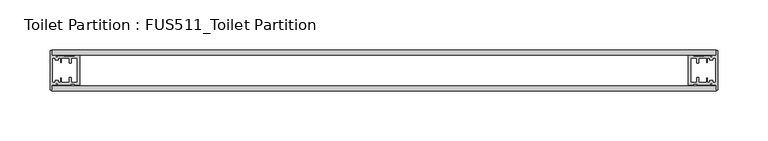
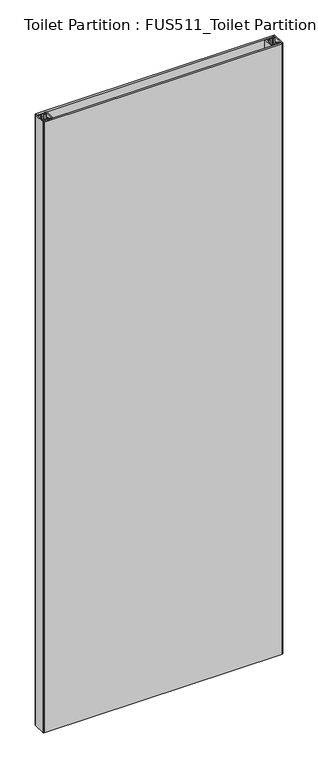
"""IFC4 building model written with IfcOpenShell, lengths in millimetres: furniture geometry, Toilet Partition : FUS511_Toilet Partition."""

from ifc_helpers import new_model, si_unit, point, frame, frame_2d, origin, place, context, project, spatial, polyline, circle_curve, trimmed, segment, composite_curve, outline, extrude, source, transform, mapped, element, save


def toilet_partition_fus511_toilet_partition_6d0bb69f(model_context):
    return source(origin(), model_context, "Body", "SweptSolid", [
        extrude(outline(composite_curve([segment(polyline([(-316.5997483, 489.5206414), (-316.5997483, 459.9080525), (-321.5351798, 459.9080525), (-321.5351798, 460.8951388), (-325.483525, 460.8951388), (-325.483525, 459.9080525), (-339.0559615, 459.9080525)]), True, "CONTINUOUS"), segment(trimmed(circle_curve(frame_2d((-339.3027331, 460.8637947)), 0.9870863), [point((-339.0559615, 459.9080525))], [point((-339.5495047, 459.9080525))], True, "CARTESIAN"), True, "CONTINUOUS"), segment(polyline([(-339.5495047, 459.9080525), (-344.2381646, 459.9080525), (-344.2381646, 454.9726211), (-345.2252509, 454.9726211)]), True, "CONTINUOUS"), segment(trimmed(circle_curve(frame_2d((-345.2252509, 455.9597074)), 0.9870863), [point((-345.2252509, 454.9726211))], [point((-346.2123372, 455.9597074))], False, "CARTESIAN"), True, "CONTINUOUS"), segment(polyline([(-346.2123372, 455.9597074), (-346.2123372, 493.4689866)]), True, "CONTINUOUS"), segment(trimmed(circle_curve(frame_2d((-345.2252509, 493.4689866)), 0.9870863), [point((-346.2123372, 493.4689866))], [point((-345.2252509, 494.4560729))], False, "CARTESIAN"), True, "CONTINUOUS"), segment(polyline([(-345.2252509, 494.4560729), (-344.2381646, 494.4560729), (-344.2381646, 489.5206414), (-339.5495047, 489.5206414)]), True, "CONTINUOUS"), segment(trimmed(circle_curve(frame_2d((-339.3027331, 488.5648992)), 0.9870863), [point((-339.5495047, 489.5206414))], [point((-339.0559615, 489.5206414))], True, "CARTESIAN"), True, "CONTINUOUS"), segment(polyline([(-339.0559615, 489.5206414), (-325.483525, 488.5335551), (-321.5351798, 488.5335551), (-321.5351798, 489.5206414), (-316.5997483, 489.5206414)]), True, "CONTINUOUS")], self_intersect=False), holes=[polyline([(-319.5610072, 486.5593825), (-324.4964387, 486.5593825), (-324.4964387, 481.623951), (-327.4576976, 481.623951), (-327.4576976, 486.5593825), (-334.3673016, 486.5593825), (-334.3673016, 482.1174942), (-335.8479311, 482.1174942), (-335.8479311, 486.5593825), (-337.5753321, 486.5593825), (-337.5753321, 484.5852099), (-341.5236773, 484.5852099), (-341.5236773, 486.5593825), (-343.2510783, 486.5593825), (-343.2510783, 462.8693114), (-341.5236773, 462.8693114), (-341.5236773, 464.843484), (-337.5753321, 464.843484), (-337.5753321, 462.8693114), (-335.8479311, 462.8693114), (-335.8479311, 467.3111998), (-334.3673016, 467.3111998), (-334.3673016, 462.8693114), (-327.4576976, 462.8693114), (-327.4576976, 467.8047429), (-324.4964387, 467.8047429), (-324.4964387, 462.8693114), (-319.5610072, 462.8693114), (-319.5610072, 486.5593825)])]), frame((0.0, 0.0, 100.0), z_axis=(0.0, 0.0, 1.0), x_axis=(1.0, 0.0, 0.0)), (0.0, 0.0, 1.0), 1800.0),
        extrude(outline(composite_curve([segment(polyline([(292.1234192, 489.5206414), (297.0588506, 489.5206414), (297.0588506, 488.5335551), (301.0071958, 488.5335551), (314.5796324, 489.5206414)]), True, "CONTINUOUS"), segment(trimmed(circle_curve(frame_2d((314.8264039, 488.5648992)), 0.9870863), [point((314.5796324, 489.5206414))], [point((315.0731755, 489.5206414))], True, "CARTESIAN"), True, "CONTINUOUS"), segment(polyline([(315.0731755, 489.5206414), (319.7618354, 489.5206414), (319.7618354, 494.4560729), (320.7489217, 494.4560729)]), True, "CONTINUOUS"), segment(trimmed(circle_curve(frame_2d((320.7489217, 493.4689866)), 0.9870863), [point((320.7489217, 494.4560729))], [point((321.736008, 493.4689866))], False, "CARTESIAN"), True, "CONTINUOUS"), segment(polyline([(321.736008, 493.4689866), (321.736008, 455.9597074)]), True, "CONTINUOUS"), segment(trimmed(circle_curve(frame_2d((320.7489217, 455.9597074)), 0.9870863), [point((321.736008, 455.9597074))], [point((320.7489217, 454.9726211))], False, "CARTESIAN"), True, "CONTINUOUS"), segment(polyline([(320.7489217, 454.9726211), (319.7618354, 454.9726211), (319.7618354, 459.9080525), (315.0731755, 459.9080525)]), True, "CONTINUOUS"), segment(trimmed(circle_curve(frame_2d((314.8264039, 460.8637947)), 0.9870863), [point((315.0731755, 459.9080525))], [point((314.5796324, 459.9080525))], True, "CARTESIAN"), True, "CONTINUOUS"), segment(polyline([(314.5796324, 459.9080525), (301.0071958, 459.9080525), (301.0071958, 460.8951388), (297.0588506, 460.8951388), (297.0588506, 459.9080525), (292.1234192, 459.9080525), (292.1234192, 489.5206414)]), True, "CONTINUOUS")], self_intersect=False), holes=[polyline([(295.084678, 486.5593825), (295.084678, 462.8693114), (300.0201095, 462.8693114), (300.0201095, 467.8047429), (302.9813684, 467.8047429), (302.9813684, 462.8693114), (309.8909725, 462.8693114), (309.8909725, 467.3111998), (311.3716019, 467.3111998), (311.3716019, 462.8693114), (313.0990029, 462.8693114), (313.0990029, 464.843484), (317.0473481, 464.843484), (317.0473481, 462.8693114), (318.7747491, 462.8693114), (318.7747491, 486.5593825), (317.0473481, 486.5593825), (317.0473481, 484.5852099), (313.0990029, 484.5852099), (313.0990029, 486.5593825), (311.3716019, 486.5593825), (311.3716019, 482.1174942), (309.8909725, 482.1174942), (309.8909725, 486.5593825), (302.9813684, 486.5593825), (302.9813684, 481.623951), (300.0201095, 481.623951), (300.0201095, 486.5593825), (295.084678, 486.5593825)])]), frame((0.0, 0.0, 100.0), z_axis=(0.0, 0.0, 1.0), x_axis=(1.0, 0.0, 0.0)), (0.0, 0.0, 1.0), 1800.0),
        extrude(outline(polyline([(-344.2381646, 454.214347), (-344.2381646, 459.214347), (319.7618354, 459.214347), (319.7618354, 454.214347), (-344.2381646, 454.214347)])), frame((0.0, 0.0, 100.0), z_axis=(0.0, 0.0, 1.0), x_axis=(1.0, 0.0, 0.0)), (0.0, 0.0, 1.0), 1800.0),
        extrude(outline(polyline([(-344.2381646, 490.214347), (-344.2381646, 495.214347), (319.7618354, 495.214347), (319.7618354, 490.214347), (-344.2381646, 490.214347)])), frame((0.0, 0.0, 100.0), z_axis=(0.0, 0.0, 1.0), x_axis=(1.0, 0.0, 0.0)), (0.0, 0.0, 1.0), 1800.0),
    ])


if __name__ == "__main__":
    model = new_model("IFC4")
    model_context = context("Model", 3, world=origin())
    ifc_project = project(units=[si_unit("LENGTHUNIT", "METRE", prefix="MILLI")], contexts=[model_context])
    site = spatial("IfcSite", under=ifc_project)
    building = spatial("IfcBuilding", under=site)
    placement = place(None, origin())
    toilet_partition_fus511_toilet_partition_shape = toilet_partition_fus511_toilet_partition_6d0bb69f(model_context)
    element("IfcFurniture", 1, ObjectType="Toilet Partition : FUS511_Toilet Partition", at=placement, inside=building, context=model_context, shape_type="MappedRepresentation", body=[
        mapped(toilet_partition_fus511_toilet_partition_shape, transform((0.0, 0.0, 0.0), x_axis=(1.0, 0.0, 0.0), y_axis=(0.0, 1.0, 0.0), z_axis=(0.0, 0.0, 1.0))),
    ])
    save(model, "model.ifc")

# Revit data of these elements
# Type "Toilet Partition : FUS511_Toilet Partition"
#   Created by = "Utku Can Kocadağ"
#   Controlled by = "Sefer Özdoğan"
#   Approved by = "Aydın Altınova"
#   Cubicle_Height = 1800 mm
#   Bot_Gap = 100 mm
#   Default Elevation = 0
# Element 1 (IfcFurniture, "Toilet Partition : FUS511_Toilet Partition")
#   Materials on its faces: "Aln_Aluminum_02"
# Materials
#   "Aln_Aluminum_02": class "Generic", colour RGB 120 120 120, transparency 0, Cost = 0
